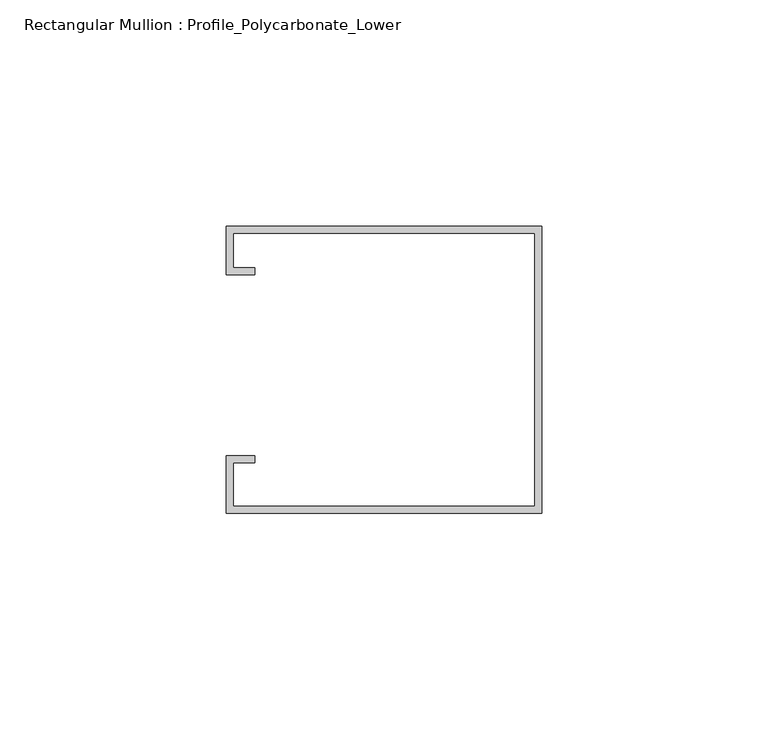
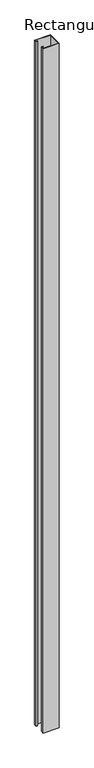
"""IFC4 building model written with IfcOpenShell, lengths in millimetres: member geometry, Rectangular Mullion : Profile_Polycarbonate_Lower."""

import ifcopenshell
import ifcopenshell.guid

model = None  # the IFC model being written
_history = None  # IfcOwnerHistory: only IFC2X3 demands one
_inside = {}  # id of a spatial element -> (the spatial element, [elements in it])
_under = {}  # id of a project, library or spatial element -> (it, [spatial elements below it])
_declared = {}  # id of a project -> (the project, [libraries it declares])
_typed = {}  # id of a type object -> (the type object, [elements of that type])
_made_of = {}  # id of a material, layer set ... -> (it, [elements and type objects made of it])


def new_model(schema):
    """Start an empty IFC model of exactly this schema.

    Asked for "IFC4X3", IfcOpenShell would pick the latest addendum, in which some entities
    have other attributes; the version numbers below select the first issue.
    IFC2X3 requires an IfcOwnerHistory on every rooted entity: one is made here for all.
    """
    global model, _history
    if schema == "IFC4X3":
        model = ifcopenshell.file(schema_version=(4, 3, 0, 0))
    else:
        model = ifcopenshell.file(schema=schema)
    _inside.clear()
    _under.clear()
    _declared.clear()
    _typed.clear()
    _made_of.clear()
    _history = None
    if model.schema == "IFC2X3":
        org = make("IfcOrganization", Name="unknown")
        user = make(
            "IfcPersonAndOrganization",
            ThePerson=make("IfcPerson", FamilyName="unknown"),
            TheOrganization=org,
        )
        app = make(
            "IfcApplication",
            ApplicationDeveloper=org,
            Version="unknown",
            ApplicationFullName="unknown",
            ApplicationIdentifier="unknown",
        )
        _history = make(
            "IfcOwnerHistory",
            OwningUser=user,
            OwningApplication=app,
            ChangeAction="ADDED",
            CreationDate=0,
        )
    return model


def make(cls, **values):
    """One entity of the class cls with the attributes given. An attribute that is None is left unset."""
    return model.create_entity(
        cls, **{name: value for name, value in values.items() if value is not None}
    )


def rooted(cls, **values):
    """An entity with a GlobalId (a new one), such as an element, a storey or a relation."""
    return make(cls, GlobalId=ifcopenshell.guid.new(), OwnerHistory=_history, **values)


def si_unit(unit_type, name, prefix=None):
    """IfcSIUnit, for example si_unit("LENGTHUNIT", "METRE", prefix="MILLI")."""
    return make("IfcSIUnit", UnitType=unit_type, Prefix=prefix, Name=name)


def assignment(units):
    """IfcUnitAssignment: the units of a project."""
    return None if units is None else make("IfcUnitAssignment", Units=units)


def point(xyz):
    """IfcCartesianPoint."""
    return None if xyz is None else make("IfcCartesianPoint", Coordinates=xyz)


def direction(xyz):
    """IfcDirection."""
    return None if xyz is None else make("IfcDirection", DirectionRatios=xyz)


def frame(location, z_axis=None, x_axis=None):
    """IfcAxis2Placement3D, a coordinate frame: its origin and axes. An axis left out is left unset."""
    return make(
        "IfcAxis2Placement3D",
        Location=point(location),
        Axis=direction(z_axis),
        RefDirection=direction(x_axis),
    )


def origin():
    """The frame at (0, 0, 0) with its axes left unset."""
    return frame((0.0, 0.0, 0.0))


def place(relative_to, where):
    """IfcLocalPlacement: puts the frame where relative to a parent placement (None: the world)."""
    return make(
        "IfcLocalPlacement", PlacementRelTo=relative_to, RelativePlacement=where
    )


def context(
    kind, dimensions, precision=None, world=None, true_north=None, identifier=None
):
    """IfcGeometricRepresentationContext, for example the 3D "Model" context."""
    return make(
        "IfcGeometricRepresentationContext",
        ContextIdentifier=identifier,
        ContextType=kind,
        CoordinateSpaceDimension=dimensions,
        Precision=precision,
        WorldCoordinateSystem=world,
        TrueNorth=true_north,
    )


def project(units=None, contexts=None):
    """IfcProject with its units and contexts."""
    return rooted(
        "IfcProject",
        Name="project",
        RepresentationContexts=contexts,
        UnitsInContext=assignment(units),
    )


def spatial(cls, under=None, at=None, **own):
    """A site, building, storey or space (cls), placed at a placement, below another one or the project."""
    s = rooted(cls, ObjectPlacement=at, **own)
    if under is not None:
        _under.setdefault(under.id(), (under, []))[1].append(s)
    return s


def polyline(points):
    """IfcPolyline through the points."""
    return make("IfcPolyline", Points=[point(p) for p in points])


def outline(outer, holes=None, kind="AREA"):
    """IfcArbitraryClosedProfileDef: a profile drawn as a closed curve; with holes, ...WithVoids."""
    if holes is None:
        return make("IfcArbitraryClosedProfileDef", ProfileType=kind, OuterCurve=outer)
    return make(
        "IfcArbitraryProfileDefWithVoids",
        ProfileType=kind,
        OuterCurve=outer,
        InnerCurves=holes,
    )


def extrude(swept, where, along, depth):
    """IfcExtrudedAreaSolid: the profile swept, set in the frame where, extruded along a direction by depth."""
    return make(
        "IfcExtrudedAreaSolid",
        SweptArea=swept,
        Position=where,
        ExtrudedDirection=direction(along),
        Depth=depth,
    )


def shape(context_of_items, identifier, shape_type, items):
    """IfcShapeRepresentation: the items that make up one representation, for example the "Body"."""
    return make(
        "IfcShapeRepresentation",
        ContextOfItems=context_of_items,
        RepresentationIdentifier=identifier,
        RepresentationType=shape_type,
        Items=items,
    )


def source(mapping_origin, context_of_items, identifier, shape_type, items):
    """IfcRepresentationMap: a shape defined once, which mapped items show again and again."""
    return make(
        "IfcRepresentationMap",
        MappingOrigin=mapping_origin,
        MappedRepresentation=shape(context_of_items, identifier, shape_type, items),
    )


def transform(
    local_origin,
    x_axis=None,
    y_axis=None,
    z_axis=None,
    scale=None,
    scale2=None,
    scale3=None,
    uniform=True,
):
    """IfcCartesianTransformationOperator3D, or its non-uniform kind. x_axis, y_axis, z_axis: its Axis1, 2, 3."""
    if uniform:
        return make(
            "IfcCartesianTransformationOperator3D",
            Axis1=direction(x_axis),
            Axis2=direction(y_axis),
            LocalOrigin=point(local_origin),
            Scale=scale,
            Axis3=direction(z_axis),
        )
    return make(
        "IfcCartesianTransformationOperator3DnonUniform",
        Axis1=direction(x_axis),
        Axis2=direction(y_axis),
        LocalOrigin=point(local_origin),
        Scale=scale,
        Axis3=direction(z_axis),
        Scale2=scale2,
        Scale3=scale3,
    )


def mapped(mapping_source, mapping_target):
    """IfcMappedItem: shows the shape of a source again, moved by a transform."""
    return make(
        "IfcMappedItem", MappingSource=mapping_source, MappingTarget=mapping_target
    )


def made_of(thing, what):
    """Note that an element or type object is made of a material, layer set ...; save() writes the relation."""
    if what is not None:
        _made_of.setdefault(what.id(), (what, []))[1].append(thing)
    return thing


def element(
    cls,
    number,
    at=None,
    inside=None,
    cuts=None,
    type_object=None,
    material=None,
    context=None,
    identifier="Body",
    shape_type=None,
    held_by="IfcProductDefinitionShape",
    body=None,
    shapes=None,
    **own,
):
    """One element of the class cls, such as IfcWall. Its Tag is "e" and its number.

    at: its placement. inside: the storey or other place that contains it. cuts: it is an
    opening in that element (IfcRelVoidsElement). A single representation is given by context,
    identifier, shape_type and body (its items); several are given by shapes. held_by: the class
    of the entity that holds the representations. save() writes the other relations.
    """
    e = rooted(cls, Tag="e%d" % number, ObjectPlacement=at, **own)
    if body is not None:
        shapes = [shape(context, identifier, shape_type, body)]
    if shapes is not None:
        e.Representation = make(held_by, Representations=shapes)
    if inside is not None:
        _inside.setdefault(inside.id(), (inside, []))[1].append(e)
    if cuts is not None:
        rooted(
            "IfcRelVoidsElement", RelatingBuildingElement=cuts, RelatedOpeningElement=e
        )
    if type_object is not None:
        _typed.setdefault(type_object.id(), (type_object, []))[1].append(e)
    return made_of(e, material)


def aggregate(whole, parts):
    """IfcRelAggregates: a whole, such as a stair, and the parts it consists of."""
    return rooted("IfcRelAggregates", RelatingObject=whole, RelatedObjects=parts)


def save(model, path):
    """Write the relations noted so far, then the file.

    IfcRelAggregates (storeys below a building ...), IfcRelContainedInSpatialStructure (elements
    in a storey), IfcRelDefinesByType, IfcRelAssociatesMaterial and IfcRelDeclares: one each for
    every whole, place, type object, material and project.
    """
    for whole, parts in _under.values():
        aggregate(whole, parts)
    for where, things in _inside.values():
        rooted(
            "IfcRelContainedInSpatialStructure",
            RelatedElements=things,
            RelatingStructure=where,
        )
    for kind, things in _typed.values():
        rooted("IfcRelDefinesByType", RelatedObjects=things, RelatingType=kind)
    for what, things in _made_of.values():
        rooted("IfcRelAssociatesMaterial", RelatedObjects=things, RelatingMaterial=what)
    for by, libraries in _declared.values():
        rooted("IfcRelDeclares", RelatingContext=by, RelatedDefinitions=libraries)
    model.write(path)


def rectangular_mullion_profile_polycarbonate_lower_46d97ac2(model_context):
    return source(origin(), model_context, "Body", "SweptSolid", [
        extrude(outline(polyline([(0.0, -32.7), (-69.85, -32.7), (-69.85, -20.0), (-63.5, -20.0), (-63.5, -21.5875), (-68.2625, -21.5875), (-68.2625, -31.1125), (-1.5875, -31.1125), (-1.5875, 29.2125), (-68.2625, 29.2125), (-68.2625, 21.5875), (-63.5, 21.5875), (-63.5, 20.0), (-69.85, 20.0), (-69.85, 30.8), (0.0, 30.8), (0.0, -32.7)])), frame((0.0, 0.0, -3149.6), z_axis=(0.0, 0.0, 1.0), x_axis=(1.0, 0.0, 0.0)), (0.0, 0.0, 1.0), 3149.6),
    ])


if __name__ == "__main__":
    model = new_model("IFC4")
    model_context = context("Model", 3, world=origin())
    ifc_project = project(units=[si_unit("LENGTHUNIT", "METRE", prefix="MILLI")], contexts=[model_context])
    site = spatial("IfcSite", under=ifc_project)
    building = spatial("IfcBuilding", under=site)
    placement = place(None, origin())
    rectangular_mullion_profile_polycarbonate_lower_shape = rectangular_mullion_profile_polycarbonate_lower_46d97ac2(model_context)
    element("IfcMember", 1, ObjectType="Rectangular Mullion : Profile_Polycarbonate_Lower", at=placement, inside=building, context=model_context, shape_type="MappedRepresentation", body=[
        mapped(rectangular_mullion_profile_polycarbonate_lower_shape, transform((0.0, 0.0, 0.0), x_axis=(1.0, 0.0, 0.0), y_axis=(0.0, 1.0, 0.0), z_axis=(0.0, 0.0, 1.0))),
    ])
    save(model, "model.ifc")

# Revit data of these elements
# Type "Rectangular Mullion : Profile_Polycarbonate_Lower"
#   built-in parameter 1007322 = 0.208333 (stored number, unit not read)
#   built-in parameter 1007321 = 0 (stored number, unit not read)
#   built-in parameter 1007320 = 0.00520833 (stored number, unit not read)
# Element 1 (IfcMember, "Rectangular Mullion : Profile_Polycarbonate_Lower")
#   Materials on its faces: "ALUMINUM PROFILE AT POLYCARBONATE PANEL"
# Materials
#   "ALUMINUM PROFILE AT POLYCARBONATE PANEL": class "Metal", colour RGB 244 244 244, transparency 0, Description = "Aluminum 6061", Cost = 0
